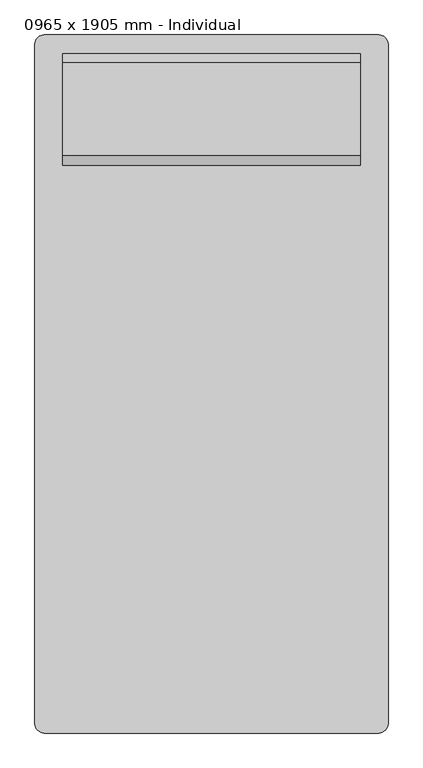
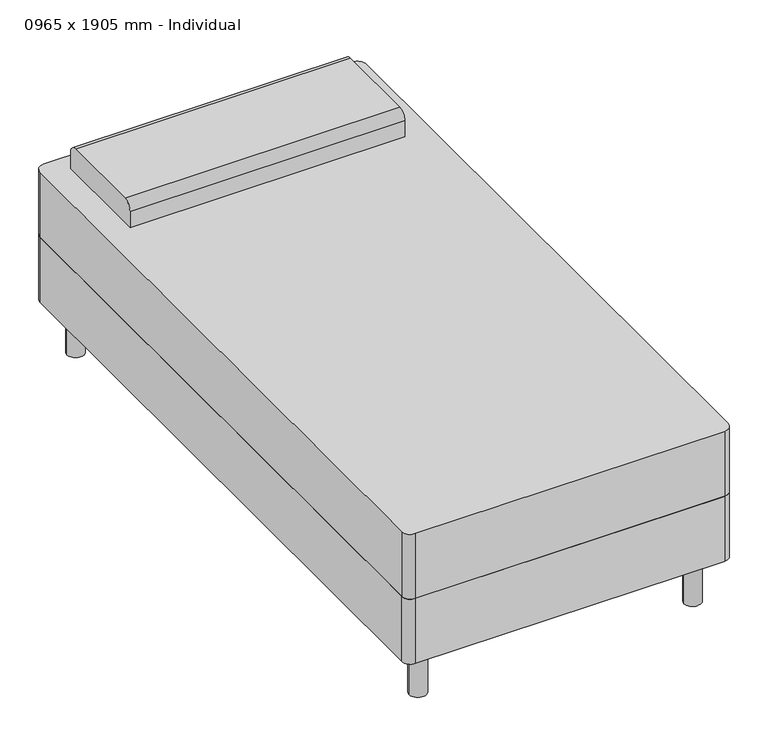
"""IFC4 building model written with IfcOpenShell, lengths in millimetres: furniture geometry, Cama-Estándar : 0965 x 1905 mm - Individual."""

from ifc_helpers import new_model, si_unit, point, frame, frame_2d, origin, origin_with_axes, place, context, project, spatial, polyline, circle_curve, trimmed, segment, composite_curve, outline, extrude, source, transform, mapped, element, save


def furniture_0965_x_1905_mm_individual_fc46863d(model_context):
    return source(origin(), model_context, "Body", "SweptSolid", [
        extrude(outline(composite_curve([segment(polyline([(-211.0114754, -972.695082), (-211.0114754, 881.504918)]), True, "CONTINUOUS"), segment(trimmed(circle_curve(frame_2d((-185.6114754, 881.504918)), 25.4), [point((-211.0114754, 881.504918))], [point((-185.6114754, 906.904918))], False, "CARTESIAN"), True, "CONTINUOUS"), segment(polyline([(-185.6114754, 906.904918), (728.5885246, 906.904918)]), True, "CONTINUOUS"), segment(trimmed(circle_curve(frame_2d((728.5885246, 881.504918)), 25.4), [point((728.5885246, 906.904918))], [point((753.9885246, 881.504918))], False, "CARTESIAN"), True, "CONTINUOUS"), segment(polyline([(753.9885246, 881.504918), (753.9885246, -972.695082)]), True, "CONTINUOUS"), segment(trimmed(circle_curve(frame_2d((728.5885246, -972.695082)), 25.4), [point((753.9885246, -972.695082))], [point((728.5885246, -998.095082))], False, "CARTESIAN"), True, "CONTINUOUS"), segment(polyline([(728.5885246, -998.095082), (-185.6114754, -998.095082)]), True, "CONTINUOUS"), segment(trimmed(circle_curve(frame_2d((-185.6114754, -972.695082)), 25.4), [point((-185.6114754, -998.095082))], [point((-211.0114754, -972.695082))], False, "CARTESIAN"), True, "CONTINUOUS")], self_intersect=False)), frame((0.0, 0.0, 152.4), z_axis=(0.0, 0.0, 1.0), x_axis=(1.0, 0.0, 0.0)), (0.0, 0.0, 1.0), 203.2),
        extrude(outline(composite_curve([segment(polyline([(551.304918, 558.8), (551.304918, 609.6)]), True, "CONTINUOUS"), segment(trimmed(circle_curve(frame_2d((576.704918, 609.6)), 25.4), [point((551.304918, 609.6))], [point((576.704918, 635.0))], False, "CARTESIAN"), True, "CONTINUOUS"), segment(polyline([(576.704918, 635.0), (830.704918, 635.0)]), True, "CONTINUOUS"), segment(trimmed(circle_curve(frame_2d((830.704918, 609.6)), 25.4), [point((830.704918, 635.0))], [point((856.104918, 609.6))], False, "CARTESIAN"), True, "CONTINUOUS"), segment(polyline([(856.104918, 609.6), (856.104918, 558.8), (551.304918, 558.8)]), True, "CONTINUOUS")], self_intersect=False)), frame((-134.8114754, 0.0, 0.0), z_axis=(1.0, 0.0, 0.0), x_axis=(0.0, 1.0, 0.0)), (0.0, 0.0, 1.0), 812.6),
        extrude(outline(composite_curve([segment(trimmed(circle_curve(frame_2d((-134.8114754, 830.704918)), 25.4), [point((-160.2114754, 830.704918))], [point((-109.4114754, 830.704918))], False, "CARTESIAN"), True, "CONTINUOUS"), segment(trimmed(circle_curve(frame_2d((-134.8114754, 830.704918)), 25.4), [point((-109.4114754, 830.704918))], [point((-160.2114754, 830.704918))], False, "CARTESIAN"), True, "CONTINUOUS")], self_intersect=False)), origin_with_axes(), (0.0, 0.0, 1.0), 152.4),
        extrude(outline(composite_curve([segment(trimmed(circle_curve(frame_2d((677.7885246, 830.704918)), 25.4), [point((652.3885246, 830.704918))], [point((703.1885246, 830.704918))], False, "CARTESIAN"), True, "CONTINUOUS"), segment(trimmed(circle_curve(frame_2d((677.7885246, 830.704918)), 25.4), [point((703.1885246, 830.704918))], [point((652.3885246, 830.704918))], False, "CARTESIAN"), True, "CONTINUOUS")], self_intersect=False)), origin_with_axes(), (0.0, 0.0, 1.0), 152.4),
        extrude(outline(composite_curve([segment(trimmed(circle_curve(frame_2d((677.7885246, -921.895082)), 25.4), [point((652.3885246, -921.895082))], [point((703.1885246, -921.895082))], False, "CARTESIAN"), True, "CONTINUOUS"), segment(trimmed(circle_curve(frame_2d((677.7885246, -921.895082)), 25.4), [point((703.1885246, -921.895082))], [point((652.3885246, -921.895082))], False, "CARTESIAN"), True, "CONTINUOUS")], self_intersect=False)), origin_with_axes(), (0.0, 0.0, 1.0), 152.4),
        extrude(outline(composite_curve([segment(trimmed(circle_curve(frame_2d((-134.8114754, -921.895082)), 25.4), [point((-160.2114754, -921.895082))], [point((-109.4114754, -921.895082))], False, "CARTESIAN"), True, "CONTINUOUS"), segment(trimmed(circle_curve(frame_2d((-134.8114754, -921.895082)), 25.4), [point((-109.4114754, -921.895082))], [point((-160.2114754, -921.895082))], False, "CARTESIAN"), True, "CONTINUOUS")], self_intersect=False)), origin_with_axes(), (0.0, 0.0, 1.0), 152.4),
        extrude(outline(composite_curve([segment(polyline([(-185.6114754, 906.904918), (728.5885246, 906.904918)]), True, "CONTINUOUS"), segment(trimmed(circle_curve(frame_2d((728.5885246, 881.504918)), 25.4), [point((728.5885246, 906.904918))], [point((753.9885246, 881.504918))], False, "CARTESIAN"), True, "CONTINUOUS"), segment(polyline([(753.9885246, 881.504918), (753.9885246, -972.695082)]), True, "CONTINUOUS"), segment(trimmed(circle_curve(frame_2d((728.5885246, -972.695082)), 25.4), [point((753.9885246, -972.695082))], [point((728.5885246, -998.095082))], False, "CARTESIAN"), True, "CONTINUOUS"), segment(polyline([(728.5885246, -998.095082), (-185.6114754, -998.095082)]), True, "CONTINUOUS"), segment(trimmed(circle_curve(frame_2d((-185.6114754, -972.695082)), 25.4), [point((-185.6114754, -998.095082))], [point((-211.0114754, -972.695082))], False, "CARTESIAN"), True, "CONTINUOUS"), segment(polyline([(-211.0114754, -972.695082), (-211.0114754, 881.504918)]), True, "CONTINUOUS"), segment(trimmed(circle_curve(frame_2d((-185.6114754, 881.504918)), 25.4), [point((-211.0114754, 881.504918))], [point((-185.6114754, 906.904918))], False, "CARTESIAN"), True, "CONTINUOUS")], self_intersect=False)), frame((0.0, 0.0, 355.6), z_axis=(0.0, 0.0, 1.0), x_axis=(1.0, 0.0, 0.0)), (0.0, 0.0, 1.0), 203.2),
    ])


if __name__ == "__main__":
    model = new_model("IFC4")
    model_context = context("Model", 3, world=origin())
    ifc_project = project(units=[si_unit("LENGTHUNIT", "METRE", prefix="MILLI")], contexts=[model_context])
    site = spatial("IfcSite", under=ifc_project)
    building = spatial("IfcBuilding", under=site)
    placement = place(None, origin())
    furniture_0965_x_1905_mm_individual_shape = furniture_0965_x_1905_mm_individual_fc46863d(model_context)
    element("IfcFurniture", 1, ObjectType="Cama-Estándar : 0965 x 1905 mm - Individual", at=placement, inside=building, context=model_context, shape_type="MappedRepresentation", body=[
        mapped(furniture_0965_x_1905_mm_individual_shape, transform((0.0, 0.0, 0.0), x_axis=(1.0, 0.0, 0.0), y_axis=(0.0, 1.0, 0.0), z_axis=(0.0, 0.0, 1.0))),
    ])
    save(model, "model.ifc")

# Revit data of these elements
# Type "Cama-Estándar : 0965 x 1905 mm - Individual"
#   Longitud = 1.905 m
#   Anchura = 0.965 m
#   Máscara [instance default] = yes
#   Material de soporte = Metal - Cromo
#   Material de colchón = Textil - Blanco
#   Default Elevation = 0
# Element 1 (IfcFurniture, "Cama-Estándar : 0965 x 1905 mm - Individual")
#   Materials on its faces: "Metal - Cromo", "Textil - Blanco"
# Materials
#   "Metal - Cromo": class "Metal", colour RGB 17 17 17, transparency 0
#   "Textil - Blanco": class "Tela", colour RGB 247 247 239, transparency 0
